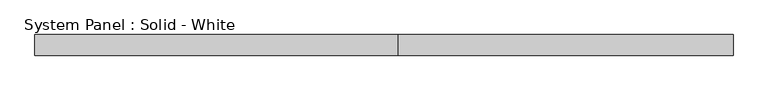
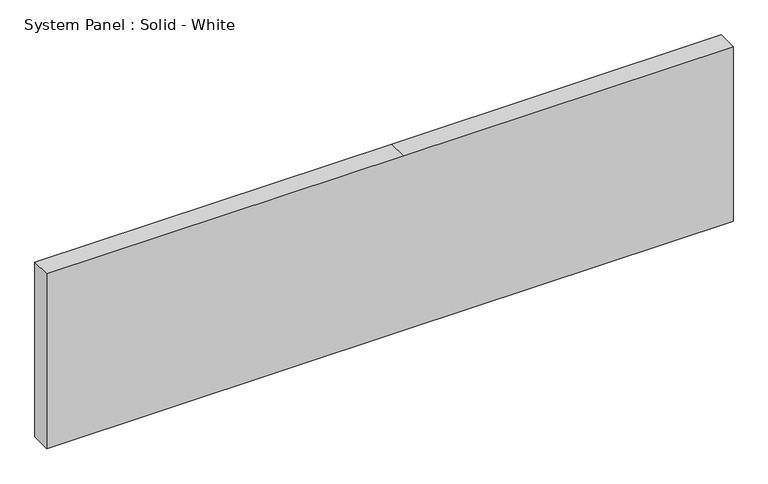
"""IFC4 building model written with IfcOpenShell, lengths in millimetres: plate geometry, System Panel : Solid - White."""

import ifcopenshell
import ifcopenshell.guid

model = None  # the IFC model being written
_history = None  # IfcOwnerHistory: only IFC2X3 demands one
_inside = {}  # id of a spatial element -> (the spatial element, [elements in it])
_under = {}  # id of a project, library or spatial element -> (it, [spatial elements below it])
_declared = {}  # id of a project -> (the project, [libraries it declares])
_typed = {}  # id of a type object -> (the type object, [elements of that type])
_made_of = {}  # id of a material, layer set ... -> (it, [elements and type objects made of it])


def new_model(schema):
    """Start an empty IFC model of exactly this schema.

    Asked for "IFC4X3", IfcOpenShell would pick the latest addendum, in which some entities
    have other attributes; the version numbers below select the first issue.
    IFC2X3 requires an IfcOwnerHistory on every rooted entity: one is made here for all.
    """
    global model, _history
    if schema == "IFC4X3":
        model = ifcopenshell.file(schema_version=(4, 3, 0, 0))
    else:
        model = ifcopenshell.file(schema=schema)
    _inside.clear()
    _under.clear()
    _declared.clear()
    _typed.clear()
    _made_of.clear()
    _history = None
    if model.schema == "IFC2X3":
        org = make("IfcOrganization", Name="unknown")
        user = make(
            "IfcPersonAndOrganization",
            ThePerson=make("IfcPerson", FamilyName="unknown"),
            TheOrganization=org,
        )
        app = make(
            "IfcApplication",
            ApplicationDeveloper=org,
            Version="unknown",
            ApplicationFullName="unknown",
            ApplicationIdentifier="unknown",
        )
        _history = make(
            "IfcOwnerHistory",
            OwningUser=user,
            OwningApplication=app,
            ChangeAction="ADDED",
            CreationDate=0,
        )
    return model


def make(cls, **values):
    """One entity of the class cls with the attributes given. An attribute that is None is left unset."""
    return model.create_entity(
        cls, **{name: value for name, value in values.items() if value is not None}
    )


def rooted(cls, **values):
    """An entity with a GlobalId (a new one), such as an element, a storey or a relation."""
    return make(cls, GlobalId=ifcopenshell.guid.new(), OwnerHistory=_history, **values)


def si_unit(unit_type, name, prefix=None):
    """IfcSIUnit, for example si_unit("LENGTHUNIT", "METRE", prefix="MILLI")."""
    return make("IfcSIUnit", UnitType=unit_type, Prefix=prefix, Name=name)


def assignment(units):
    """IfcUnitAssignment: the units of a project."""
    return None if units is None else make("IfcUnitAssignment", Units=units)


def point(xyz):
    """IfcCartesianPoint."""
    return None if xyz is None else make("IfcCartesianPoint", Coordinates=xyz)


def direction(xyz):
    """IfcDirection."""
    return None if xyz is None else make("IfcDirection", DirectionRatios=xyz)


def frame(location, z_axis=None, x_axis=None):
    """IfcAxis2Placement3D, a coordinate frame: its origin and axes. An axis left out is left unset."""
    return make(
        "IfcAxis2Placement3D",
        Location=point(location),
        Axis=direction(z_axis),
        RefDirection=direction(x_axis),
    )


def origin():
    """The frame at (0, 0, 0) with its axes left unset."""
    return frame((0.0, 0.0, 0.0))


def place(relative_to, where):
    """IfcLocalPlacement: puts the frame where relative to a parent placement (None: the world)."""
    return make(
        "IfcLocalPlacement", PlacementRelTo=relative_to, RelativePlacement=where
    )


def context(
    kind, dimensions, precision=None, world=None, true_north=None, identifier=None
):
    """IfcGeometricRepresentationContext, for example the 3D "Model" context."""
    return make(
        "IfcGeometricRepresentationContext",
        ContextIdentifier=identifier,
        ContextType=kind,
        CoordinateSpaceDimension=dimensions,
        Precision=precision,
        WorldCoordinateSystem=world,
        TrueNorth=true_north,
    )


def project(units=None, contexts=None):
    """IfcProject with its units and contexts."""
    return rooted(
        "IfcProject",
        Name="project",
        RepresentationContexts=contexts,
        UnitsInContext=assignment(units),
    )


def spatial(cls, under=None, at=None, **own):
    """A site, building, storey or space (cls), placed at a placement, below another one or the project."""
    s = rooted(cls, ObjectPlacement=at, **own)
    if under is not None:
        _under.setdefault(under.id(), (under, []))[1].append(s)
    return s


def polyline(points):
    """IfcPolyline through the points."""
    return make("IfcPolyline", Points=[point(p) for p in points])


def outline(outer, holes=None, kind="AREA"):
    """IfcArbitraryClosedProfileDef: a profile drawn as a closed curve; with holes, ...WithVoids."""
    if holes is None:
        return make("IfcArbitraryClosedProfileDef", ProfileType=kind, OuterCurve=outer)
    return make(
        "IfcArbitraryProfileDefWithVoids",
        ProfileType=kind,
        OuterCurve=outer,
        InnerCurves=holes,
    )


def extrude(swept, where, along, depth):
    """IfcExtrudedAreaSolid: the profile swept, set in the frame where, extruded along a direction by depth."""
    return make(
        "IfcExtrudedAreaSolid",
        SweptArea=swept,
        Position=where,
        ExtrudedDirection=direction(along),
        Depth=depth,
    )


def shape(context_of_items, identifier, shape_type, items):
    """IfcShapeRepresentation: the items that make up one representation, for example the "Body"."""
    return make(
        "IfcShapeRepresentation",
        ContextOfItems=context_of_items,
        RepresentationIdentifier=identifier,
        RepresentationType=shape_type,
        Items=items,
    )


def source(mapping_origin, context_of_items, identifier, shape_type, items):
    """IfcRepresentationMap: a shape defined once, which mapped items show again and again."""
    return make(
        "IfcRepresentationMap",
        MappingOrigin=mapping_origin,
        MappedRepresentation=shape(context_of_items, identifier, shape_type, items),
    )


def transform(
    local_origin,
    x_axis=None,
    y_axis=None,
    z_axis=None,
    scale=None,
    scale2=None,
    scale3=None,
    uniform=True,
):
    """IfcCartesianTransformationOperator3D, or its non-uniform kind. x_axis, y_axis, z_axis: its Axis1, 2, 3."""
    if uniform:
        return make(
            "IfcCartesianTransformationOperator3D",
            Axis1=direction(x_axis),
            Axis2=direction(y_axis),
            LocalOrigin=point(local_origin),
            Scale=scale,
            Axis3=direction(z_axis),
        )
    return make(
        "IfcCartesianTransformationOperator3DnonUniform",
        Axis1=direction(x_axis),
        Axis2=direction(y_axis),
        LocalOrigin=point(local_origin),
        Scale=scale,
        Axis3=direction(z_axis),
        Scale2=scale2,
        Scale3=scale3,
    )


def mapped(mapping_source, mapping_target):
    """IfcMappedItem: shows the shape of a source again, moved by a transform."""
    return make(
        "IfcMappedItem", MappingSource=mapping_source, MappingTarget=mapping_target
    )


def made_of(thing, what):
    """Note that an element or type object is made of a material, layer set ...; save() writes the relation."""
    if what is not None:
        _made_of.setdefault(what.id(), (what, []))[1].append(thing)
    return thing


def element(
    cls,
    number,
    at=None,
    inside=None,
    cuts=None,
    type_object=None,
    material=None,
    context=None,
    identifier="Body",
    shape_type=None,
    held_by="IfcProductDefinitionShape",
    body=None,
    shapes=None,
    **own,
):
    """One element of the class cls, such as IfcWall. Its Tag is "e" and its number.

    at: its placement. inside: the storey or other place that contains it. cuts: it is an
    opening in that element (IfcRelVoidsElement). A single representation is given by context,
    identifier, shape_type and body (its items); several are given by shapes. held_by: the class
    of the entity that holds the representations. save() writes the other relations.
    """
    e = rooted(cls, Tag="e%d" % number, ObjectPlacement=at, **own)
    if body is not None:
        shapes = [shape(context, identifier, shape_type, body)]
    if shapes is not None:
        e.Representation = make(held_by, Representations=shapes)
    if inside is not None:
        _inside.setdefault(inside.id(), (inside, []))[1].append(e)
    if cuts is not None:
        rooted(
            "IfcRelVoidsElement", RelatingBuildingElement=cuts, RelatedOpeningElement=e
        )
    if type_object is not None:
        _typed.setdefault(type_object.id(), (type_object, []))[1].append(e)
    return made_of(e, material)


def aggregate(whole, parts):
    """IfcRelAggregates: a whole, such as a stair, and the parts it consists of."""
    return rooted("IfcRelAggregates", RelatingObject=whole, RelatedObjects=parts)


def save(model, path):
    """Write the relations noted so far, then the file.

    IfcRelAggregates (storeys below a building ...), IfcRelContainedInSpatialStructure (elements
    in a storey), IfcRelDefinesByType, IfcRelAssociatesMaterial and IfcRelDeclares: one each for
    every whole, place, type object, material and project.
    """
    for whole, parts in _under.values():
        aggregate(whole, parts)
    for where, things in _inside.values():
        rooted(
            "IfcRelContainedInSpatialStructure",
            RelatedElements=things,
            RelatingStructure=where,
        )
    for kind, things in _typed.values():
        rooted("IfcRelDefinesByType", RelatedObjects=things, RelatingType=kind)
    for what, things in _made_of.values():
        rooted("IfcRelAssociatesMaterial", RelatedObjects=things, RelatingMaterial=what)
    for by, libraries in _declared.values():
        rooted("IfcRelDeclares", RelatingContext=by, RelatedDefinitions=libraries)
    model.write(path)


def system_panel_solid_white_5cb61f8d(model_context):
    return source(origin(), model_context, "Body", "SweptSolid", [
        extrude(outline(polyline([(0.0, -1073.6035714), (0.0, 43.0892857), (0.0, 1073.6035714), (577.85, 1073.6035714), (577.85, 43.0892857), (577.85, -1073.6035714), (0.0, -1073.6035714)])), frame((0.0, -19.05, 0.0), z_axis=(0.0, 1.0, 0.0), x_axis=(0.0, 0.0, 1.0)), (0.0, 0.0, 1.0), 63.5),
    ])


if __name__ == "__main__":
    model = new_model("IFC4")
    model_context = context("Model", 3, world=origin())
    ifc_project = project(units=[si_unit("LENGTHUNIT", "METRE", prefix="MILLI")], contexts=[model_context])
    site = spatial("IfcSite", under=ifc_project)
    building = spatial("IfcBuilding", under=site)
    placement = place(None, origin())
    system_panel_solid_white_shape = system_panel_solid_white_5cb61f8d(model_context)
    element("IfcPlate", 1, ObjectType="System Panel : Solid - White", at=placement, inside=building, context=model_context, shape_type="MappedRepresentation", body=[
        mapped(system_panel_solid_white_shape, transform((0.0, 0.0, 0.0), x_axis=(1.0, 0.0, 0.0), y_axis=(0.0, 1.0, 0.0), z_axis=(0.0, 0.0, 1.0))),
    ])
    save(model, "model.ifc")

# Revit data of these elements
# Element 1 (IfcPlate, "System Panel : Solid - White")
#   Materials on its faces: "White Panel"
# Materials
#   "White Panel": class "Unassigned", colour RGB 255 255 255, transparency 0
